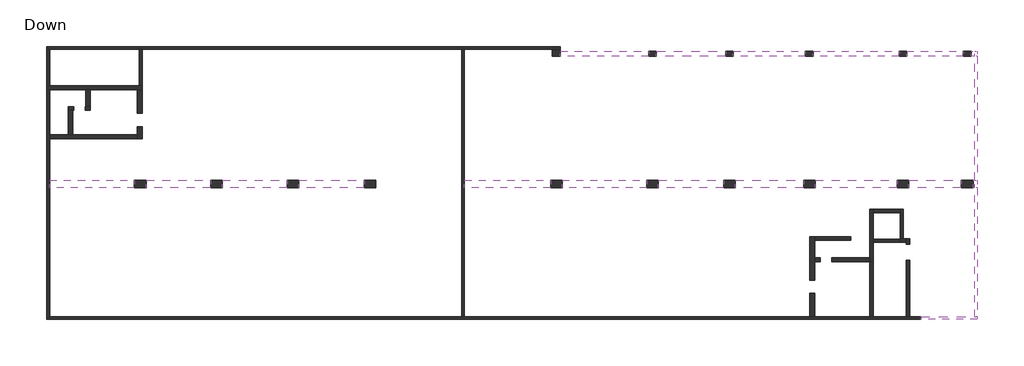
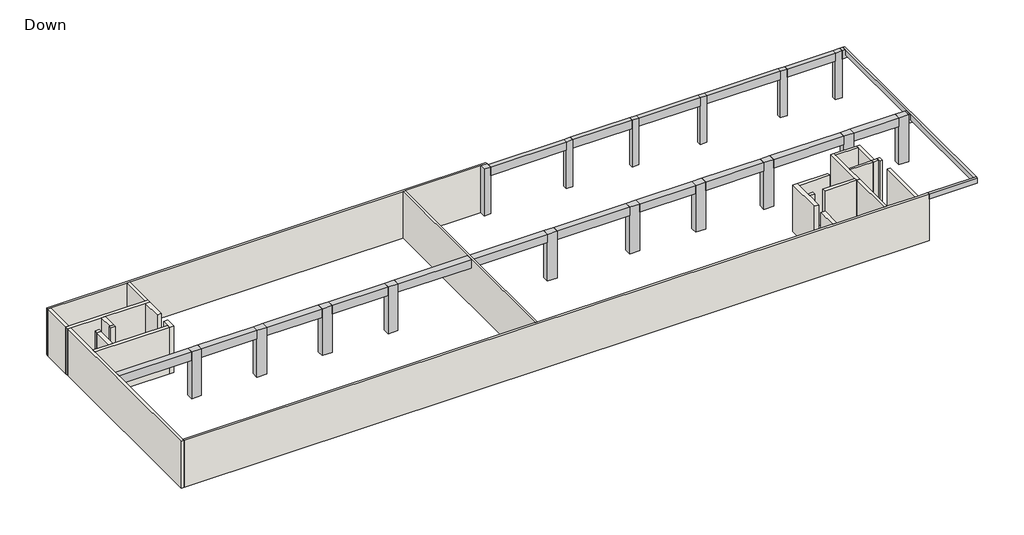
# One storey: 27 walls, 19 beams, 16 columns.
"""IFC4 building model written with IfcOpenShell, lengths in millimetres."""

from ifc_helpers import new_model, si_unit, frame, origin, origin_with_axes, place, context, project, spatial, polyline, outline, extrude, faceted_brep, element, save

model = new_model("IFC4")

# Units and contexts
model_context = context("Model", 3, world=origin())
ifc_project = project(units=[si_unit("LENGTHUNIT", "METRE", prefix="MILLI")], contexts=[model_context])

# Site, building, storey
site = spatial("IfcSite", under=ifc_project)
building = spatial("IfcBuilding", under=site)
storey = spatial("IfcBuildingStorey", under=building, Name="Down", Elevation=0.0)

# Beams
placement = place(None, origin())
element("IfcBeam", 1, ObjectType="Concrete Rectengular Beam : 20/50", at=placement, inside=storey, context=model_context, shape_type="Brep", body=[
    faceted_brep([(30873.6352373, -8183.3289062, 4500.0), (30873.6352373, -8183.3289062, 4000.0), (30873.6352373, -8383.3289062, 4000.0), (30873.6352373, -8383.3289062, 4500.0), (35273.6352373, -8383.3289062, 4500.0), (35273.6352373, -8183.3289062, 4500.0), (35073.6352373, -8183.3289062, 4500.0), (35273.6352373, -8383.3289062, 4000.0), (35073.6352373, -8183.3289062, 4000.0), (35273.6352373, -8183.3289062, 4000.0)], [[[0, 1, 2, 3]], [[0, 3, 4, 5, 6]], [[3, 2, 7, 4]], [[2, 1, 8, 9, 7]], [[1, 0, 6, 5, 9, 8]], [[5, 4, 7, 9]]]),
])
element("IfcBeam", 2, ObjectType="Concrete Rectengular Beam : 20/50", at=placement, inside=storey, context=model_context, shape_type="Brep", body=[
    faceted_brep([(35273.6352373, 12515.9833477, 4500.0), (35073.6352373, 12515.9833477, 4500.0), (35073.6352373, 12115.9833477, 4500.0), (35073.6352373, 2452.6133039, 4500.0), (35073.6352373, 1852.6133039, 4500.0), (35073.6352373, -8183.3289062, 4500.0), (35273.6352373, -8183.3289062, 4500.0), (35273.6352373, 12515.9833477, 4000.0), (35273.6352373, -8183.3289062, 4000.0), (35273.6352373, 1852.6133039, 4000.0), (35273.6352373, 2452.6133039, 4000.0), (35273.6352373, 12115.9833477, 4000.0), (35073.6352373, 12515.9833477, 4000.0), (35073.6352373, -8183.3289062, 4000.0), (35073.6352373, 1852.6133039, 4000.0), (35073.6352373, 2452.6133039, 4000.0), (35073.6352373, 12115.9833477, 4000.0), (35073.6352373, -8183.3289062, 4100.0)], [[[0, 1, 2, 3, 4, 5, 6]], [[7, 0, 6, 8, 9, 10, 11]], [[12, 7, 11, 10, 9, 8, 13, 14, 15, 16]], [[1, 12, 16, 15, 14, 13, 17, 5, 4, 3, 2]], [[1, 0, 7, 12]], [[6, 5, 17, 13, 8]]]),
])
element("IfcBeam", 3, ObjectType="Concrete Rectengular Beam : 40/80", at=placement, inside=storey, context=model_context, shape_type="Brep", body=[
    faceted_brep([(34777.3208435, 12515.9833477, 4500.0), (34777.3208435, 12115.9833477, 4500.0), (35073.6352373, 12115.9833477, 4500.0), (35073.6352373, 12515.9833477, 4500.0), (35273.6352373, 12515.9833477, 3700.0), (34777.3208435, 12515.9833477, 3700.0), (35073.6352373, 12515.9833477, 4000.0), (35273.6352373, 12515.9833477, 4000.0), (35273.6352373, 12115.9833477, 3700.0), (34777.3208435, 12115.9833477, 3700.0), (35273.6352373, 12115.9833477, 4000.0), (35073.6352373, 12115.9833477, 4000.0), (35073.6352373, 12115.9833477, 4100.0), (34777.3208435, 12115.9833477, 4100.0)], [[[0, 1, 2, 3]], [[4, 5, 0, 3, 6, 7]], [[4, 8, 9, 5]], [[9, 8, 10, 11, 12, 2, 1, 13]], [[8, 4, 7, 10]], [[1, 0, 5, 9, 13]], [[6, 11, 10, 7]], [[11, 6, 3, 2, 12]]]),
])
element("IfcBeam", 4, ObjectType="Concrete Rectengular Beam : 40/80", at=placement, inside=storey, context=model_context, shape_type="Brep", body=[
    faceted_brep([(29770.3049975, 12515.9833477, 4500.0), (29770.3049975, 12115.9833477, 4500.0), (34177.3208435, 12115.9833477, 4500.0), (34177.3208435, 12515.9833477, 4500.0), (29770.3049975, 12515.9833477, 3700.0), (34177.3208435, 12515.9833477, 3700.0), (29770.3049975, 12115.9833477, 3700.0), (34177.3208435, 12115.9833477, 3700.0), (29770.3049975, 12115.9833477, 4100.0), (34177.3208435, 12115.9833477, 4100.0)], [[[0, 1, 2, 3]], [[4, 0, 3, 5]], [[6, 4, 5, 7]], [[2, 1, 8, 6, 7, 9]], [[1, 0, 4, 6, 8]], [[3, 2, 9, 7, 5]]]),
])
element("IfcBeam", 5, ObjectType="Concrete Rectengular Beam : 40/80", at=placement, inside=storey, context=model_context, shape_type="Brep", body=[
    faceted_brep([(22477.3114752, 12515.9833477, 4500.0), (22477.3114752, 12115.9833477, 4500.0), (29170.3049975, 12115.9833477, 4500.0), (29170.3049975, 12515.9833477, 4500.0), (22477.3114752, 12515.9833477, 3700.0), (29170.3049975, 12515.9833477, 3700.0), (22477.3114752, 12115.9833477, 3700.0), (29170.3049975, 12115.9833477, 3700.0), (22477.3114752, 12115.9833477, 4100.0), (29170.3049975, 12115.9833477, 4100.0)], [[[0, 1, 2, 3]], [[4, 0, 3, 5]], [[6, 4, 5, 7]], [[2, 1, 8, 6, 7, 9]], [[1, 0, 4, 6, 8]], [[3, 2, 9, 7, 5]]]),
])
element("IfcBeam", 6, ObjectType="Concrete Rectengular Beam : 40/80", at=placement, inside=storey, context=model_context, shape_type="Brep", body=[
    faceted_brep([(21877.3114752, 12115.9833477, 4500.0), (21877.3114752, 12515.9833477, 4500.0), (16270.7293524, 12515.9833477, 4500.0), (16270.7293524, 12115.9833477, 4500.0), (21877.3114752, 12515.9833477, 3700.0), (16270.7293524, 12515.9833477, 3700.0), (21877.3114752, 12115.9833477, 3700.0), (16270.7293524, 12115.9833477, 3700.0), (16270.7293524, 12115.9833477, 4100.0), (21877.3114752, 12115.9833477, 4100.0)], [[[0, 1, 2, 3]], [[1, 4, 5, 2]], [[4, 6, 7, 5]], [[0, 3, 8, 7, 6, 9]], [[1, 0, 9, 6, 4]], [[3, 2, 5, 7, 8]]]),
])
element("IfcBeam", 7, ObjectType="Concrete Rectengular Beam : 40/80", at=placement, inside=storey, context=model_context, shape_type="Brep", body=[
    faceted_brep([(15670.7293524, 12115.9833477, 4500.0), (15670.7293524, 12515.9833477, 4500.0), (10272.0355776, 12515.9833477, 4500.0), (10272.0355776, 12115.9833477, 4500.0), (15670.7293524, 12515.9833477, 3700.0), (10272.0355776, 12515.9833477, 3700.0), (15670.7293524, 12115.9833477, 3700.0), (10272.0355776, 12115.9833477, 3700.0), (10272.0355776, 12115.9833477, 4100.0), (15670.7293524, 12115.9833477, 4100.0)], [[[0, 1, 2, 3]], [[1, 4, 5, 2]], [[4, 6, 7, 5]], [[0, 3, 8, 7, 6, 9]], [[1, 0, 9, 6, 4]], [[3, 2, 5, 7, 8]]]),
])
element("IfcBeam", 8, ObjectType="Concrete Rectengular Beam : 40/80", at=placement, inside=storey, context=model_context, shape_type="Brep", body=[
    faceted_brep([(9672.0355776, 12115.9833477, 4500.0), (9672.0355776, 12515.9833477, 4500.0), (2774.3455353, 12515.9833477, 4500.0), (2774.3455353, 12115.9833477, 4500.0), (9672.0355776, 12515.9833477, 3700.0), (2774.3455353, 12515.9833477, 3700.0), (9672.0355776, 12115.9833477, 3700.0), (2774.3455353, 12115.9833477, 3700.0), (2774.3455353, 12115.9833477, 4100.0), (9672.0355776, 12115.9833477, 4100.0)], [[[0, 1, 2, 3]], [[1, 4, 5, 2]], [[4, 6, 7, 5]], [[0, 3, 8, 7, 6, 9]], [[1, 0, 9, 6, 4]], [[3, 2, 5, 7, 8]]]),
])
element("IfcBeam", 9, ObjectType="Concrete Rectengular Beam : 60/80", at=placement, inside=storey, context=model_context, shape_type="Brep", body=[
    faceted_brep([(34927.3208435, 2452.6133039, 4500.0), (34927.3208435, 1852.6133039, 4500.0), (35073.6352373, 1852.6133039, 4500.0), (35073.6352373, 2452.6133039, 4500.0), (34927.3208435, 1852.6133039, 3700.0), (35273.6352373, 1852.6133039, 3700.0), (35273.6352373, 1852.6133039, 4000.0), (35073.6352373, 1852.6133039, 4000.0), (35073.6352373, 1852.6133039, 4100.0), (35273.6352373, 2452.6133039, 3700.0), (34927.3208435, 2452.6133039, 3700.0), (35073.6352373, 2452.6133039, 4100.0), (35073.6352373, 2452.6133039, 4000.0), (35273.6352373, 2452.6133039, 4000.0)], [[[0, 1, 2, 3]], [[4, 5, 6, 7, 8, 2, 1]], [[9, 5, 4, 10]], [[9, 10, 0, 3, 11, 12, 13]], [[5, 9, 13, 6]], [[1, 0, 10, 4]], [[12, 7, 6, 13]], [[7, 12, 11, 3, 2, 8]]]),
])
element("IfcBeam", 10, ObjectType="Concrete Rectengular Beam : 60/80", at=placement, inside=storey, context=model_context, shape_type="SweptSolid", body=[
    extrude(outline(polyline([(29920.3049975, 1852.6133039), (29920.3049975, 2452.6133039), (34027.3208435, 2452.6133039), (34027.3208435, 1852.6133039), (29920.3049975, 1852.6133039)])), frame((0.0, 0.0, 3700.0), z_axis=(0.0, 0.0, 1.0), x_axis=(1.0, 0.0, 0.0)), (0.0, 0.0, 1.0), 800.0),
])
element("IfcBeam", 11, ObjectType="Concrete Rectengular Beam : 60/80", at=placement, inside=storey, context=model_context, shape_type="SweptSolid", body=[
    extrude(outline(polyline([(29020.3049975, 2452.6133039), (29020.3049975, 1852.6133039), (22627.3114752, 1852.6133039), (22627.3114752, 2452.6133039), (29020.3049975, 2452.6133039)])), frame((0.0, 0.0, 3700.0), z_axis=(0.0, 0.0, 1.0), x_axis=(1.0, 0.0, 0.0)), (0.0, 0.0, 1.0), 800.0),
])
element("IfcBeam", 12, ObjectType="Concrete Rectengular Beam : 60/80", at=placement, inside=storey, context=model_context, shape_type="SweptSolid", body=[
    extrude(outline(polyline([(21727.3114752, 2452.6133039), (21727.3114752, 1852.6133039), (16420.7293524, 1852.6133039), (16420.7293524, 2452.6133039), (21727.3114752, 2452.6133039)])), frame((0.0, 0.0, 3700.0), z_axis=(0.0, 0.0, 1.0), x_axis=(1.0, 0.0, 0.0)), (0.0, 0.0, 1.0), 800.0),
])
element("IfcBeam", 13, ObjectType="Concrete Rectengular Beam : 60/80", at=placement, inside=storey, context=model_context, shape_type="SweptSolid", body=[
    extrude(outline(polyline([(15520.7293524, 2452.6133039), (15520.7293524, 1852.6133039), (10422.0355776, 1852.6133039), (10422.0355776, 2452.6133039), (15520.7293524, 2452.6133039)])), frame((0.0, 0.0, 3700.0), z_axis=(0.0, 0.0, 1.0), x_axis=(1.0, 0.0, 0.0)), (0.0, 0.0, 1.0), 800.0),
])
element("IfcBeam", 14, ObjectType="Concrete Rectengular Beam : 60/80", at=placement, inside=storey, context=model_context, shape_type="SweptSolid", body=[
    extrude(outline(polyline([(9522.0355776, 2452.6133039), (9522.0355776, 1852.6133039), (2924.3455353, 1852.6133039), (2924.3455353, 2452.6133039), (9522.0355776, 2452.6133039)])), frame((0.0, 0.0, 3700.0), z_axis=(0.0, 0.0, 1.0), x_axis=(1.0, 0.0, 0.0)), (0.0, 0.0, 1.0), 800.0),
])
element("IfcBeam", 15, ObjectType="Concrete Rectengular Beam : 60/80", at=placement, inside=storey, context=model_context, shape_type="Brep", body=[
    faceted_brep([(-11589.7528998, 2452.6133039, 4500.0), (-11589.7528998, 1852.6133039, 4500.0), (-4886.1401685, 1852.6133039, 4500.0), (-4886.1401685, 2452.6133039, 4500.0), (-11589.7528998, 2452.6133039, 3700.0), (-4886.1401685, 2452.6133039, 4100.0), (-4886.1401685, 2452.6133039, 3700.0), (-11589.7528998, 1852.6133039, 3700.0), (-4886.1401685, 1852.6133039, 3700.0), (-4886.1401685, 1852.6133039, 4100.0)], [[[0, 1, 2, 3]], [[4, 0, 3, 5, 6]], [[7, 4, 6, 8]], [[1, 7, 8, 9, 2]], [[1, 0, 4, 7]], [[3, 2, 9, 8, 6, 5]]]),
    faceted_brep([(2024.3455353, 2452.6133039, 4500.0), (2024.3455353, 1852.6133039, 4500.0), (2024.3455353, 1852.6133039, 3700.0), (2024.3455353, 2452.6133039, 3700.0), (-4686.1401685, 1852.6133039, 4500.0), (-4686.1401685, 2452.6133039, 4500.0), (-4686.1401685, 2452.6133039, 4100.0), (-4686.1401685, 2452.6133039, 3700.0), (-4686.1401685, 1852.6133039, 3700.0), (-4686.1401685, 1852.6133039, 4100.0)], [[[0, 1, 2, 3]], [[4, 5, 6, 7, 8, 9]], [[1, 0, 5, 4]], [[0, 3, 7, 6, 5]], [[3, 2, 8, 7]], [[2, 1, 4, 9, 8]]]),
])
element("IfcBeam", 16, ObjectType="Concrete Rectengular Beam : 60/80", at=placement, inside=storey, context=model_context, shape_type="SweptSolid", body=[
    extrude(outline(polyline([(-12489.7528998, 2452.6133039), (-12489.7528998, 1852.6133039), (-17591.3777818, 1852.6133039), (-17591.3777818, 2452.6133039), (-12489.7528998, 2452.6133039)])), frame((0.0, 0.0, 3700.0), z_axis=(0.0, 0.0, 1.0), x_axis=(1.0, 0.0, 0.0)), (0.0, 0.0, 1.0), 800.0),
])
element("IfcBeam", 17, ObjectType="Concrete Rectengular Beam : 60/80", at=placement, inside=storey, context=model_context, shape_type="SweptSolid", body=[
    extrude(outline(polyline([(-18491.3777818, 2452.6133039), (-18491.3777818, 1852.6133039), (-23534.5891488, 1852.6133039), (-23534.5891488, 2452.6133039), (-18491.3777818, 2452.6133039)])), frame((0.0, 0.0, 3700.0), z_axis=(0.0, 0.0, 1.0), x_axis=(1.0, 0.0, 0.0)), (0.0, 0.0, 1.0), 800.0),
])
element("IfcBeam", 18, ObjectType="Concrete Rectengular Beam : 60/80", at=placement, inside=storey, context=model_context, shape_type="SweptSolid", body=[
    extrude(outline(polyline([(-24434.5891488, 2452.6133039), (-24434.5891488, 1852.6133039), (-29484.6297539, 1852.6133039), (-29484.6297539, 2452.6133039), (-24434.5891488, 2452.6133039)])), frame((0.0, 0.0, 3700.0), z_axis=(0.0, 0.0, 1.0), x_axis=(1.0, 0.0, 0.0)), (0.0, 0.0, 1.0), 800.0),
])
element("IfcBeam", 19, ObjectType="Concrete Rectengular Beam : 60/80", at=placement, inside=storey, context=model_context, shape_type="Brep", body=[
    faceted_brep([(-30384.6297539, 1852.6133039, 4500.0), (-30384.6297539, 2452.6133039, 4500.0), (-36981.5324359, 2452.6133039, 4500.0), (-36981.5324359, 1852.6133039, 4500.0), (-30384.6297539, 2452.6133039, 3700.0), (-36981.5324359, 2452.6133039, 3700.0), (-36981.5324359, 2452.6133039, 4100.0), (-30384.6297539, 1852.6133039, 3700.0), (-36981.5324359, 1852.6133039, 3700.0), (-36981.5324359, 1852.6133039, 4100.0)], [[[0, 1, 2, 3]], [[1, 4, 5, 6, 2]], [[4, 7, 8, 5]], [[7, 0, 3, 9, 8]], [[1, 0, 7, 4]], [[3, 2, 6, 5, 8, 9]]]),
])

# Columns
element("IfcColumn", 20, ObjectType="Concrete Rectengular Column : 40/60", at=placement, inside=storey, context=model_context, shape_type="SweptSolid", body=[
    extrude(outline(polyline([(21877.3114752, 12515.9833477), (22477.3114752, 12515.9833477), (22477.3114752, 12115.9833477), (21877.3114752, 12115.9833477), (21877.3114752, 12515.9833477)])), origin_with_axes(), (0.0, 0.0, 1.0), 4500.0),
])
element("IfcColumn", 21, ObjectType="Concrete Rectengular Column : 40/60", at=placement, inside=storey, context=model_context, shape_type="SweptSolid", body=[
    extrude(outline(polyline([(15670.7293524, 12515.9833477), (16270.7293524, 12515.9833477), (16270.7293524, 12115.9833477), (15670.7293524, 12115.9833477), (15670.7293524, 12515.9833477)])), origin_with_axes(), (0.0, 0.0, 1.0), 4500.0),
])
element("IfcColumn", 22, ObjectType="Concrete Rectengular Column : 40/60", at=placement, inside=storey, context=model_context, shape_type="SweptSolid", body=[
    extrude(outline(polyline([(9672.0355776, 12515.9833477), (10272.0355776, 12515.9833477), (10272.0355776, 12115.9833477), (9672.0355776, 12115.9833477), (9672.0355776, 12515.9833477)])), origin_with_axes(), (0.0, 0.0, 1.0), 4500.0),
])
element("IfcColumn", 23, ObjectType="Concrete Rectengular Column : 40/60", at=placement, inside=storey, context=model_context, shape_type="SweptSolid", body=[
    extrude(outline(polyline([(29770.3049975, 12115.9833477), (29170.3049975, 12115.9833477), (29170.3049975, 12515.9833477), (29770.3049975, 12515.9833477), (29770.3049975, 12115.9833477)])), origin_with_axes(), (0.0, 0.0, 1.0), 4500.0),
])
element("IfcColumn", 24, ObjectType="Concrete Rectengular Column : 40/60", at=placement, inside=storey, context=model_context, shape_type="SweptSolid", body=[
    extrude(outline(polyline([(34777.3208435, 12115.9833477), (34177.3208435, 12115.9833477), (34177.3208435, 12515.9833477), (34777.3208435, 12515.9833477), (34777.3208435, 12115.9833477)])), origin_with_axes(), (0.0, 0.0, 1.0), 4500.0),
])
element("IfcColumn", 25, ObjectType="Concrete Rectengular Column : 55/60", at=placement, inside=storey, context=model_context, shape_type="Brep", body=[
    faceted_brep([(2174.3455353, 12665.9833477, 0.0), (2774.3455353, 12665.9833477, 0.0), (2774.3455353, 12115.9833477, 0.0), (2174.3455353, 12115.9833477, 0.0), (2174.3455353, 12665.9833477, 4500.0), (2774.3455353, 12665.9833477, 4500.0), (2174.3455353, 12665.9833477, 4100.0), (2774.3455353, 12115.9833477, 4500.0), (2174.3455353, 12115.9833477, 4500.0), (2174.3455353, 12115.9833477, 4100.0)], [[[0, 1, 2, 3]], [[4, 5, 1, 0, 6]], [[5, 7, 2, 1]], [[7, 8, 9, 3, 2]], [[8, 4, 6, 0, 3, 9]], [[4, 8, 7, 5]]]),
])
element("IfcColumn", 26, ObjectType="Concrete Rectengular Column : 60/90", at=placement, inside=storey, context=model_context, shape_type="SweptSolid", body=[
    extrude(outline(polyline([(29020.3049975, 2452.6133039), (29920.3049975, 2452.6133039), (29920.3049975, 1852.6133039), (29020.3049975, 1852.6133039), (29020.3049975, 2452.6133039)])), origin_with_axes(), (0.0, 0.0, 1.0), 4500.0),
])
element("IfcColumn", 27, ObjectType="Concrete Rectengular Column : 60/90", at=placement, inside=storey, context=model_context, shape_type="SweptSolid", body=[
    extrude(outline(polyline([(34027.3208435, 2452.6133039), (34927.3208435, 2452.6133039), (34927.3208435, 1852.6133039), (34027.3208435, 1852.6133039), (34027.3208435, 2452.6133039)])), origin_with_axes(), (0.0, 0.0, 1.0), 4500.0),
])
element("IfcColumn", 28, ObjectType="Concrete Rectengular Column : 60/90", at=placement, inside=storey, context=model_context, shape_type="SweptSolid", body=[
    extrude(outline(polyline([(21727.3114752, 2452.6133039), (22627.3114752, 2452.6133039), (22627.3114752, 1852.6133039), (21727.3114752, 1852.6133039), (21727.3114752, 2452.6133039)])), origin_with_axes(), (0.0, 0.0, 1.0), 4500.0),
])
element("IfcColumn", 29, ObjectType="Concrete Rectengular Column : 60/90", at=placement, inside=storey, context=model_context, shape_type="SweptSolid", body=[
    extrude(outline(polyline([(15520.7293524, 2452.6133039), (16420.7293524, 2452.6133039), (16420.7293524, 1852.6133039), (15520.7293524, 1852.6133039), (15520.7293524, 2452.6133039)])), origin_with_axes(), (0.0, 0.0, 1.0), 4500.0),
])
element("IfcColumn", 30, ObjectType="Concrete Rectengular Column : 60/90", at=placement, inside=storey, context=model_context, shape_type="SweptSolid", body=[
    extrude(outline(polyline([(9522.0355776, 2452.6133039), (10422.0355776, 2452.6133039), (10422.0355776, 1852.6133039), (9522.0355776, 1852.6133039), (9522.0355776, 2452.6133039)])), origin_with_axes(), (0.0, 0.0, 1.0), 4500.0),
])
element("IfcColumn", 31, ObjectType="Concrete Rectengular Column : 60/90", at=placement, inside=storey, context=model_context, shape_type="SweptSolid", body=[
    extrude(outline(polyline([(2024.3455353, 2452.6133039), (2924.3455353, 2452.6133039), (2924.3455353, 1852.6133039), (2024.3455353, 1852.6133039), (2024.3455353, 2452.6133039)])), origin_with_axes(), (0.0, 0.0, 1.0), 4500.0),
])
element("IfcColumn", 32, ObjectType="Concrete Rectengular Column : 60/90", at=placement, inside=storey, context=model_context, shape_type="SweptSolid", body=[
    extrude(outline(polyline([(-12489.7528998, 2452.6133039), (-11589.7528998, 2452.6133039), (-11589.7528998, 1852.6133039), (-12489.7528998, 1852.6133039), (-12489.7528998, 2452.6133039)])), origin_with_axes(), (0.0, 0.0, 1.0), 4500.0),
])
element("IfcColumn", 33, ObjectType="Concrete Rectengular Column : 60/90", at=placement, inside=storey, context=model_context, shape_type="SweptSolid", body=[
    extrude(outline(polyline([(-18491.3777818, 2452.6133039), (-17591.3777818, 2452.6133039), (-17591.3777818, 1852.6133039), (-18491.3777818, 1852.6133039), (-18491.3777818, 2452.6133039)])), origin_with_axes(), (0.0, 0.0, 1.0), 4500.0),
])
element("IfcColumn", 34, ObjectType="Concrete Rectengular Column : 60/90", at=placement, inside=storey, context=model_context, shape_type="SweptSolid", body=[
    extrude(outline(polyline([(-24434.5891488, 2452.6133039), (-23534.5891488, 2452.6133039), (-23534.5891488, 1852.6133039), (-24434.5891488, 1852.6133039), (-24434.5891488, 2452.6133039)])), origin_with_axes(), (0.0, 0.0, 1.0), 4500.0),
])
element("IfcColumn", 35, ObjectType="Concrete Rectengular Column : 60/90", at=placement, inside=storey, context=model_context, shape_type="SweptSolid", body=[
    extrude(outline(polyline([(-30384.6297539, 2452.6133039), (-29484.6297539, 2452.6133039), (-29484.6297539, 1852.6133039), (-30384.6297539, 1852.6133039), (-30384.6297539, 2452.6133039)])), origin_with_axes(), (0.0, 0.0, 1.0), 4500.0),
])

# Walls
element("IfcWall", 36, ObjectType="20", at=placement, inside=storey, context=model_context, shape_type="Brep", body=[
    faceted_brep([(2774.3455353, 12865.9833477, 0.0), (-37231.5324359, 12865.9833477, 0.0), (-37231.5324359, 12865.9833477, 4500.0), (2774.3455353, 12865.9833477, 4500.0), (2774.3455353, 12665.9833477, 0.0), (2774.3455353, 12665.9833477, 4500.0), (2174.3455353, 12665.9833477, 4500.0), (-4686.1401685, 12665.9833477, 4500.0), (-4886.1401685, 12665.9833477, 4500.0), (-29780.4573498, 12665.9833477, 4500.0), (-30010.4573498, 12665.9833477, 4500.0), (-36981.5324359, 12665.9833477, 4500.0), (-37231.5324359, 12665.9833477, 4500.0), (-37231.5324359, 12665.9833477, 0.0), (-36981.5324359, 12665.9833477, 0.0), (-30010.4573498, 12665.9833477, 0.0), (-29780.4573498, 12665.9833477, 0.0), (-4886.1401685, 12665.9833477, 0.0), (-4686.1401685, 12665.9833477, 0.0), (2174.3455353, 12665.9833477, 0.0)], [[[0, 1, 2, 3]], [[4, 5, 6, 7, 8, 9, 10, 11, 12, 13, 14, 15, 16, 17, 18, 19]], [[1, 0, 4, 19, 18, 17, 16, 15, 14, 13]], [[3, 2, 12, 11, 10, 9, 8, 7, 6, 5]], [[0, 3, 5, 4]], [[2, 1, 13, 12]]]),
])
element("IfcWall", 37, ObjectType="20", at=placement, inside=storey, context=model_context, shape_type="Brep", body=[
    faceted_brep([(-36981.5324359, -8383.3289062, 0.0), (30873.6352373, -8383.3289062, 0.0), (30873.6352373, -8383.3289062, 4000.0), (30873.6352373, -8383.3289062, 4500.0), (-36981.5324359, -8383.3289062, 4500.0), (-36981.5324359, -8183.3289062, 0.0), (-36981.5324359, -8183.3289062, 4100.0), (-36981.5324359, -8183.3289062, 4500.0), (-4886.1401685, -8183.3289062, 4500.0), (-4686.1401685, -8183.3289062, 4500.0), (22192.8106957, -8183.3289062, 4500.0), (22592.8106957, -8183.3289062, 4500.0), (26893.3884, -8183.3289062, 4500.0), (27143.3884, -8183.3289062, 4500.0), (29744.7199004, -8183.3289062, 4500.0), (29994.7199004, -8183.3289062, 4500.0), (30873.6352373, -8183.3289062, 4500.0), (30873.6352373, -8183.3289062, 4000.0), (30873.6352373, -8183.3289062, 0.0), (29994.7199004, -8183.3289062, 0.0), (29744.7199004, -8183.3289062, 0.0), (27143.3884, -8183.3289062, 0.0), (26893.3884, -8183.3289062, 0.0), (22592.8106957, -8183.3289062, 0.0), (22192.8106957, -8183.3289062, 0.0), (-4686.1401685, -8183.3289062, 0.0), (-4886.1401685, -8183.3289062, 0.0)], [[[0, 1, 2, 3, 4]], [[5, 6, 7, 8, 9, 10, 11, 12, 13, 14, 15, 16, 17, 18, 19, 20, 21, 22, 23, 24, 25, 26]], [[1, 0, 5, 26, 25, 24, 23, 22, 21, 20, 19, 18]], [[3, 2, 1, 18, 17, 16]], [[4, 3, 16, 15, 14, 13, 12, 11, 10, 9, 8, 7]], [[0, 4, 7, 6, 5]]]),
])
element("IfcWall", 38, ObjectType="20", at=placement, inside=storey, context=model_context, shape_type="SweptSolid", body=[
    extrude(outline(polyline([(27139.9357672, -2160.3079756), (29245.3524403, -2160.3079756), (29245.3524403, -2360.3079756), (27139.9357672, -2360.3079756), (27139.9357672, -2160.3079756)])), origin_with_axes(), (0.0, 0.0, 1.0), 4500.0),
])
element("IfcWall", 39, ObjectType="20", at=placement, inside=storey, context=model_context, shape_type="Brep", body=[
    faceted_brep([(-4886.1401685, 12665.9833477, 0.0), (-4886.1401685, -8183.3289062, 0.0), (-4886.1401685, -8183.3289062, 4100.0), (-4886.1401685, -8183.3289062, 4500.0), (-4886.1401685, 1852.6133039, 4500.0), (-4886.1401685, 2452.6133039, 4500.0), (-4886.1401685, 12665.9833477, 4500.0), (-4886.1401685, 12665.9833477, 4100.0), (-4686.1401685, 12665.9833477, 0.0), (-4686.1401685, 12665.9833477, 4100.0), (-4686.1401685, 12665.9833477, 4500.0), (-4686.1401685, 2452.6133039, 4500.0), (-4686.1401685, 1852.6133039, 4500.0), (-4686.1401685, -8183.3289062, 4500.0), (-4686.1401685, -8183.3289062, 4100.0), (-4686.1401685, -8183.3289062, 0.0)], [[[0, 1, 2, 3, 4, 5, 6, 7]], [[8, 9, 10, 11, 12, 13, 14, 15]], [[1, 0, 8, 15]], [[6, 5, 4, 3, 13, 12, 11, 10]], [[0, 7, 6, 10, 9, 8]], [[3, 2, 1, 15, 14, 13]]]),
])
element("IfcWall", 40, ObjectType="23", at=placement, inside=storey, context=model_context, shape_type="Brep", body=[
    faceted_brep([(-30010.4573498, 12665.9833477, 0.0), (-30010.4573498, 9800.978884, 0.0), (-30010.4573498, 9800.978884, 4500.0), (-30010.4573498, 12665.9833477, 4500.0), (-29780.4573498, 12665.9833477, 0.0), (-29780.4573498, 12665.9833477, 4100.0), (-29780.4573498, 12665.9833477, 4500.0), (-29780.4573498, 9800.978884, 4500.0), (-29780.4573498, 9800.978884, 0.0)], [[[0, 1, 2, 3]], [[4, 5, 6, 7, 8]], [[1, 0, 4, 8]], [[3, 2, 7, 6]], [[0, 3, 6, 5, 4]], [[2, 1, 8, 7]]]),
])
element("IfcWall", 41, ObjectType="25", at=placement, inside=storey, context=model_context, shape_type="SweptSolid", body=[
    extrude(outline(polyline([(-36981.5324359, 12665.9833477), (-36981.5324359, 9800.978884), (-37231.5324359, 9800.978884), (-37231.5324359, 12665.9833477), (-36981.5324359, 12665.9833477)])), origin_with_axes(), (0.0, 0.0, 1.0), 4500.0),
])
element("IfcWall", 42, ObjectType="25", at=placement, inside=storey, context=model_context, shape_type="Brep", body=[
    faceted_brep([(-37231.5324359, 9500.978884, 0.0), (-37231.5324359, -8383.3289062, 0.0), (-37231.5324359, -8383.3289062, 4500.0), (-37231.5324359, 9500.978884, 4500.0), (-36981.5324359, 9500.978884, 0.0), (-36981.5324359, 9500.978884, 4250.0), (-36981.5324359, 9500.978884, 4500.0), (-36981.5324359, 5997.6022486, 4500.0), (-36981.5324359, 5697.6022486, 4500.0), (-36981.5324359, 2452.6133039, 4500.0), (-36981.5324359, 1852.6133039, 4500.0), (-36981.5324359, -8183.3289062, 4500.0), (-36981.5324359, -8383.3289062, 4500.0), (-36981.5324359, -8383.3289062, 0.0), (-36981.5324359, -8183.3289062, 0.0), (-36981.5324359, 5697.6022486, 0.0), (-36981.5324359, 5997.6022486, 0.0)], [[[0, 1, 2, 3]], [[4, 5, 6, 7, 8, 9, 10, 11, 12, 13, 14, 15, 16]], [[1, 0, 4, 16, 15, 14, 13]], [[3, 2, 12, 11, 10, 9, 8, 7, 6]], [[0, 3, 6, 5, 4]], [[2, 1, 13, 12]]]),
])
element("IfcWall", 43, ObjectType="25", at=placement, inside=storey, context=model_context, shape_type="Brep", body=[
    faceted_brep([(29994.7199004, -8183.3289062, 0.0), (29994.7199004, -3766.5105737, 0.0), (29994.7199004, -3766.5105737, 4100.0), (29994.7199004, -3766.5105737, 4500.0), (29994.7199004, -8183.3289062, 4500.0), (29994.7199004, -8183.3289062, 4100.0), (29744.7199004, -8183.3289062, 0.0), (29744.7199004, -8183.3289062, 4500.0), (29744.7199004, -3766.5105737, 4500.0), (29744.7199004, -3766.5105737, 4100.0), (29744.7199004, -3766.5105737, 0.0)], [[[0, 1, 2, 3, 4, 5]], [[6, 7, 8, 9, 10]], [[1, 0, 6, 10]], [[3, 2, 1, 10, 9, 8]], [[4, 3, 8, 7]], [[0, 5, 4, 7, 6]]]),
])
element("IfcWall", 44, ObjectType="25", at=placement, inside=storey, context=model_context, shape_type="Brep", body=[
    faceted_brep([(29994.7199004, -2514.5866947, 0.0), (29994.7199004, -2110.3079756, 0.0), (29994.7199004, -2110.3079756, 4100.0), (29994.7199004, -2110.3079756, 4500.0), (29994.7199004, -2514.5866947, 4500.0), (29994.7199004, -2514.5866947, 4100.0), (29744.7199004, -2514.5866947, 0.0), (29744.7199004, -2514.5866947, 4100.0), (29744.7199004, -2514.5866947, 4500.0), (29744.7199004, -2360.3079756, 4500.0), (29744.7199004, -2110.3079756, 4500.0), (29744.7199004, -2110.3079756, 0.0), (29744.7199004, -2360.3079756, 0.0)], [[[0, 1, 2, 3, 4, 5]], [[6, 7, 8, 9, 10, 11, 12]], [[1, 0, 6, 12, 11]], [[4, 3, 10, 9, 8]], [[0, 5, 4, 8, 7, 6]], [[3, 2, 1, 11, 10]]]),
])
element("IfcWall", 45, ObjectType="25", at=placement, inside=storey, context=model_context, shape_type="Brep", body=[
    faceted_brep([(29744.7199004, -2110.3079756, 0.0), (29495.5138576, -2110.3079756, 0.0), (29245.5138576, -2110.3079756, 0.0), (29245.3524403, -2110.3079756, 0.0), (29245.3524403, -2110.3079756, 4500.0), (29245.5138576, -2110.3079756, 4500.0), (29495.5138576, -2110.3079756, 4500.0), (29744.7199004, -2110.3079756, 4500.0), (29744.7199004, -2360.3079756, 0.0), (29744.7199004, -2360.3079756, 4500.0), (29245.3524403, -2360.3079756, 4500.0), (29245.3524403, -2360.3079756, 0.0), (29245.3524403, -2160.3079756, 0.0), (29245.3524403, -2160.3079756, 4500.0)], [[[0, 1, 2, 3, 4, 5, 6, 7]], [[8, 9, 10, 11]], [[3, 2, 1, 0, 8, 11, 12]], [[4, 3, 12, 11, 10, 13]], [[7, 6, 5, 4, 13, 10, 9]], [[0, 7, 9, 8]]]),
])
element("IfcWall", 46, ObjectType="25", at=placement, inside=storey, context=model_context, shape_type="Brep", body=[
    faceted_brep([(29495.5138576, -2110.3079756, 0.0), (29495.5138576, 189.1668387, 0.0), (29495.5138576, 189.1668387, 4100.0), (29495.5138576, 189.1668387, 4500.0), (29495.5138576, -2110.3079756, 4500.0), (29495.5138576, -2110.3079756, 4100.0), (29245.5138576, -2110.3079756, 0.0), (29245.5138576, -2110.3079756, 4500.0), (29245.5138576, -60.8331613, 4500.0), (29245.5138576, 189.1668387, 4500.0), (29245.5138576, 189.1668387, 0.0), (29245.5138576, -60.8331613, 0.0)], [[[0, 1, 2, 3, 4, 5]], [[6, 7, 8, 9, 10, 11]], [[1, 0, 6, 11, 10]], [[4, 3, 9, 8, 7]], [[0, 5, 4, 7, 6]], [[3, 2, 1, 10, 9]]]),
])
element("IfcWall", 47, ObjectType="25", at=placement, inside=storey, context=model_context, shape_type="SweptSolid", body=[
    extrude(outline(polyline([(27139.9357672, 189.1668387), (29245.5138576, 189.1668387), (29245.5138576, -60.8331613), (27139.9357672, -60.8331613), (27139.9357672, 189.1668387)])), origin_with_axes(), (0.0, 0.0, 1.0), 4500.0),
])
element("IfcWall", 48, ObjectType="25", at=placement, inside=storey, context=model_context, shape_type="Brep", body=[
    faceted_brep([(26893.3884, -3883.3566788, 0.0), (26893.3884, -8183.3289062, 0.0), (26893.3884, -8183.3289062, 4250.0), (26893.3884, -8183.3289062, 4500.0), (26893.3884, -3883.3566788, 4500.0), (26893.3884, -3883.3566788, 4250.0), (27143.3884, -3883.3566788, 0.0), (27143.3884, -3883.3566788, 4500.0), (27143.3884, -8183.3289062, 4500.0), (27143.3884, -8183.3289062, 0.0), (27139.9357672, -3883.3566788, 0.0), (27139.9357672, -3883.3566788, 4500.0)], [[[0, 1, 2, 3, 4, 5]], [[6, 7, 8, 9]], [[1, 0, 10, 6, 9]], [[4, 3, 8, 7, 11]], [[0, 5, 4, 11, 7, 6, 10]], [[3, 2, 1, 9, 8]]]),
])
element("IfcWall", 49, ObjectType="27", at=placement, inside=storey, context=model_context, shape_type="Brep", body=[
    faceted_brep([(26869.9357672, 189.1668387, 0.0), (26869.9357672, -3583.3566788, 0.0), (26869.9357672, -3883.3566788, 0.0), (26869.9357672, -3883.3566788, 4500.0), (26869.9357672, -3583.3566788, 4500.0), (26869.9357672, -1932.7380409, 4500.0), (26869.9357672, 189.1668387, 4500.0), (26869.9357672, 189.1668387, 4100.0), (27139.9357672, 189.1668387, 0.0), (27139.9357672, 189.1668387, 4500.0), (27139.9357672, -60.8331613, 4500.0), (27139.9357672, -2160.3079756, 4500.0), (27139.9357672, -2360.3079756, 4500.0), (27139.9357672, -3883.3566788, 4500.0), (27139.9357672, -3883.3566788, 0.0), (27139.9357672, -2360.3079756, 0.0), (27139.9357672, -2160.3079756, 0.0), (27139.9357672, -60.8331613, 0.0), (26893.3884, -3883.3566788, 0.0), (26893.3884, -3883.3566788, 4500.0)], [[[0, 1, 2, 3, 4, 5, 6, 7]], [[8, 9, 10, 11, 12, 13, 14, 15, 16, 17]], [[2, 1, 0, 8, 17, 16, 15, 14, 18]], [[6, 5, 4, 3, 19, 13, 12, 11, 10, 9]], [[0, 7, 6, 9, 8]], [[3, 2, 18, 14, 13, 19]]]),
])
element("IfcWall", 50, ObjectType="27", at=placement, inside=storey, context=model_context, shape_type="Brep", body=[
    faceted_brep([(-35525.2356133, 7897.529186, 0.0), (-35175.2356133, 7897.529186, 0.0), (-35131.0080225, 7897.529186, 0.0), (-35131.0080225, 7897.529186, 4250.0), (-35131.0080225, 7897.529186, 4500.0), (-35175.2356133, 7897.529186, 4500.0), (-35525.2356133, 7897.529186, 4500.0), (-35525.2356133, 8167.529186, 0.0), (-35525.2356133, 8167.529186, 4250.0), (-35525.2356133, 8167.529186, 4500.0), (-35131.0080225, 8167.529186, 4500.0), (-35131.0080225, 8167.529186, 4250.0), (-35131.0080225, 8167.529186, 0.0)], [[[0, 1, 2, 3, 4, 5, 6]], [[7, 8, 9, 10, 11, 12]], [[2, 1, 0, 7, 12]], [[4, 3, 2, 12, 11, 10]], [[6, 5, 4, 10, 9]], [[0, 6, 9, 8, 7]]]),
])
element("IfcWall", 51, ObjectType="27", at=placement, inside=storey, context=model_context, shape_type="Brep", body=[
    faceted_brep([(-34230.8736368, 7897.529186, 0.0), (-33829.9452937, 7897.529186, 0.0), (-33829.9452937, 7897.529186, 4250.0), (-33829.9452937, 7897.529186, 4500.0), (-34230.8736368, 7897.529186, 4500.0), (-34230.8736368, 7897.529186, 4250.0), (-34230.8736368, 8167.529186, 0.0), (-34230.8736368, 8167.529186, 4250.0), (-34230.8736368, 8167.529186, 4500.0), (-34179.9452937, 8167.529186, 4500.0), (-33829.9452937, 8167.529186, 4500.0), (-33829.9452937, 8167.529186, 0.0), (-34179.9452937, 8167.529186, 0.0)], [[[0, 1, 2, 3, 4, 5]], [[6, 7, 8, 9, 10, 11, 12]], [[1, 0, 6, 12, 11]], [[4, 3, 10, 9, 8]], [[0, 5, 4, 8, 7, 6]], [[3, 2, 1, 11, 10]]]),
])
element("IfcWall", 52, ObjectType="30", at=placement, inside=storey, context=model_context, shape_type="Brep", body=[
    faceted_brep([(-29780.4573498, 9800.978884, 0.0), (-30010.4573498, 9800.978884, 0.0), (-36981.5324359, 9800.978884, 0.0), (-37231.5324359, 9800.978884, 0.0), (-37231.5324359, 9800.978884, 4500.0), (-36981.5324359, 9800.978884, 4500.0), (-30010.4573498, 9800.978884, 4500.0), (-29780.4573498, 9800.978884, 4500.0), (-29780.4573498, 9500.978884, 0.0), (-29780.4573498, 9500.978884, 4500.0), (-30180.4573498, 9500.978884, 4500.0), (-33829.9452937, 9500.978884, 4500.0), (-34179.9452937, 9500.978884, 4500.0), (-36981.5324359, 9500.978884, 4500.0), (-37231.5324359, 9500.978884, 4500.0), (-37231.5324359, 9500.978884, 0.0), (-36981.5324359, 9500.978884, 0.0), (-34179.9452937, 9500.978884, 0.0), (-33829.9452937, 9500.978884, 0.0), (-30180.4573498, 9500.978884, 0.0)], [[[0, 1, 2, 3, 4, 5, 6, 7]], [[8, 9, 10, 11, 12, 13, 14, 15, 16, 17, 18, 19]], [[3, 2, 1, 0, 8, 19, 18, 17, 16, 15]], [[7, 6, 5, 4, 14, 13, 12, 11, 10, 9]], [[4, 3, 15, 14]], [[0, 7, 9, 8]]]),
])
element("IfcWall", 53, ObjectType="30", at=placement, inside=storey, context=model_context, shape_type="Brep", body=[
    faceted_brep([(25386.8359355, -1932.7380409, 0.0), (22592.8106957, -1932.7380409, 0.0), (22592.8106957, -1932.7380409, 4500.0), (25386.8359355, -1932.7380409, 4500.0), (25386.8359355, -1932.7380409, 4250.0), (25386.8359355, -2232.7380409, 0.0), (25386.8359355, -2232.7380409, 4250.0), (25386.8359355, -2232.7380409, 4500.0), (22592.8106957, -2232.7380409, 4500.0), (22592.8106957, -2232.7380409, 4250.0), (22592.8106957, -2232.7380409, 0.0)], [[[0, 1, 2, 3, 4]], [[5, 6, 7, 8, 9, 10]], [[1, 0, 5, 10]], [[3, 2, 8, 7]], [[0, 4, 3, 7, 6, 5]], [[2, 1, 10, 9, 8]]]),
])
element("IfcWall", 54, ObjectType="30", at=placement, inside=storey, context=model_context, shape_type="Brep", body=[
    faceted_brep([(22592.8106957, -3883.3566788, 0.0), (23037.1054794, -3883.3566788, 0.0), (23037.1054794, -3883.3566788, 4250.0), (23037.1054794, -3883.3566788, 4500.0), (22592.8106957, -3883.3566788, 4500.0), (22592.8106957, -3883.3566788, 4250.0), (22592.8106957, -3583.3566788, 0.0), (22592.8106957, -3583.3566788, 4250.0), (22592.8106957, -3583.3566788, 4500.0), (23037.1054794, -3583.3566788, 4500.0), (23037.1054794, -3583.3566788, 4250.0), (23037.1054794, -3583.3566788, 0.0), (23037.1054794, -3733.3566788, 4500.0)], [[[0, 1, 2, 3, 4, 5]], [[6, 7, 8, 9, 10, 11]], [[1, 0, 6, 11]], [[3, 2, 1, 11, 10, 9, 12]], [[4, 3, 12, 9, 8]], [[0, 5, 4, 8, 7, 6]]]),
])
element("IfcWall", 55, ObjectType="30", at=placement, inside=storey, context=model_context, shape_type="Brep", body=[
    faceted_brep([(23943.9406174, -3883.3566788, 0.0), (26869.9357672, -3883.3566788, 0.0), (26869.9357672, -3883.3566788, 4500.0), (23943.9406174, -3883.3566788, 4500.0), (23943.9406174, -3883.3566788, 4250.0), (23943.9406174, -3583.3566788, 0.0), (23943.9406174, -3583.3566788, 4250.0), (23943.9406174, -3583.3566788, 4500.0), (26869.9357672, -3583.3566788, 4500.0), (26869.9357672, -3583.3566788, 4250.0), (26869.9357672, -3583.3566788, 0.0), (23943.9406174, -3733.3566788, 4500.0)], [[[0, 1, 2, 3, 4]], [[5, 6, 7, 8, 9, 10]], [[1, 0, 5, 10]], [[3, 2, 8, 7, 11]], [[0, 4, 3, 11, 7, 6, 5]], [[2, 1, 10, 9, 8]]]),
])
element("IfcWall", 56, ObjectType="30", at=placement, inside=storey, context=model_context, shape_type="Brep", body=[
    faceted_brep([(-36981.5324359, 5697.6022486, 0.0), (-30180.4573498, 5697.6022486, 0.0), (-30180.4573498, 5697.6022486, 4500.0), (-36981.5324359, 5697.6022486, 4500.0), (-36981.5324359, 5697.6022486, 4100.0), (-36981.5324359, 5997.6022486, 0.0), (-36981.5324359, 5997.6022486, 4250.0), (-36981.5324359, 5997.6022486, 4500.0), (-35525.2356133, 5997.6022486, 4500.0), (-35175.2356133, 5997.6022486, 4500.0), (-30180.4573498, 5997.6022486, 4500.0), (-30180.4573498, 5997.6022486, 4250.0), (-30180.4573498, 5997.6022486, 0.0), (-35175.2356133, 5997.6022486, 0.0), (-35525.2356133, 5997.6022486, 0.0)], [[[0, 1, 2, 3, 4]], [[5, 6, 7, 8, 9, 10, 11, 12, 13, 14]], [[1, 0, 5, 14, 13, 12]], [[3, 2, 10, 9, 8, 7]], [[0, 4, 3, 7, 6, 5]], [[2, 1, 12, 11, 10]]]),
])
element("IfcWall", 57, ObjectType="35", at=placement, inside=storey, context=model_context, shape_type="Brep", body=[
    faceted_brep([(-35175.2356133, 5997.6022486, 0.0), (-35175.2356133, 7897.529186, 0.0), (-35175.2356133, 7897.529186, 4250.0), (-35175.2356133, 7897.529186, 4500.0), (-35175.2356133, 5997.6022486, 4500.0), (-35175.2356133, 5997.6022486, 4250.0), (-35525.2356133, 5997.6022486, 0.0), (-35525.2356133, 5997.6022486, 4250.0), (-35525.2356133, 5997.6022486, 4500.0), (-35525.2356133, 7897.529186, 4500.0), (-35525.2356133, 7897.529186, 0.0)], [[[0, 1, 2, 3, 4, 5]], [[6, 7, 8, 9, 10]], [[1, 0, 6, 10]], [[4, 3, 9, 8]], [[0, 5, 4, 8, 7, 6]], [[3, 2, 1, 10, 9]]]),
])
element("IfcWall", 58, ObjectType="35", at=placement, inside=storey, context=model_context, shape_type="Brep", body=[
    faceted_brep([(-33829.9452937, 8167.529186, 0.0), (-33829.9452937, 9500.978884, 0.0), (-33829.9452937, 9500.978884, 4250.0), (-33829.9452937, 9500.978884, 4500.0), (-33829.9452937, 8167.529186, 4500.0), (-34179.9452937, 8167.529186, 0.0), (-34179.9452937, 8167.529186, 4250.0), (-34179.9452937, 8167.529186, 4500.0), (-34179.9452937, 9500.978884, 4500.0), (-34179.9452937, 9500.978884, 4250.0), (-34179.9452937, 9500.978884, 0.0)], [[[0, 1, 2, 3, 4]], [[5, 6, 7, 8, 9, 10]], [[1, 0, 5, 10]], [[4, 3, 8, 7]], [[0, 4, 7, 6, 5]], [[3, 2, 1, 10, 9, 8]]]),
])
element("IfcWall", 59, ObjectType="40", at=placement, inside=storey, context=model_context, shape_type="Brep", body=[
    faceted_brep([(22192.8106957, -1932.7380409, 0.0), (22192.8106957, -5323.3186801, 0.0), (22192.8106957, -5323.3186801, 4100.0), (22192.8106957, -5323.3186801, 4500.0), (22192.8106957, -1932.7380409, 4500.0), (22192.8106957, -1932.7380409, 4100.0), (22592.8106957, -1932.7380409, 0.0), (22592.8106957, -1932.7380409, 4500.0), (22592.8106957, -2232.7380409, 4500.0), (22592.8106957, -3583.3566788, 4500.0), (22592.8106957, -3883.3566788, 4500.0), (22592.8106957, -5323.3186801, 4500.0), (22592.8106957, -5323.3186801, 4100.0), (22592.8106957, -5323.3186801, 0.0), (22592.8106957, -3883.3566788, 0.0), (22592.8106957, -3583.3566788, 0.0), (22592.8106957, -2232.7380409, 0.0)], [[[0, 1, 2, 3, 4, 5]], [[6, 7, 8, 9, 10, 11, 12, 13, 14, 15, 16]], [[1, 0, 6, 16, 15, 14, 13]], [[3, 2, 1, 13, 12, 11]], [[4, 3, 11, 10, 9, 8, 7]], [[0, 5, 4, 7, 6]]]),
])
element("IfcWall", 60, ObjectType="40", at=placement, inside=storey, context=model_context, shape_type="Brep", body=[
    faceted_brep([(22192.8106957, -6342.9498143, 0.0), (22192.8106957, -8183.3289062, 0.0), (22192.8106957, -8183.3289062, 4100.0), (22192.8106957, -8183.3289062, 4500.0), (22192.8106957, -6342.9498143, 4500.0), (22192.8106957, -6342.9498143, 4100.0), (22592.8106957, -6342.9498143, 0.0), (22592.8106957, -6342.9498143, 4100.0), (22592.8106957, -6342.9498143, 4500.0), (22592.8106957, -8183.3289062, 4500.0), (22592.8106957, -8183.3289062, 4250.0), (22592.8106957, -8183.3289062, 0.0)], [[[0, 1, 2, 3, 4, 5]], [[6, 7, 8, 9, 10, 11]], [[1, 0, 6, 11]], [[4, 3, 9, 8]], [[0, 5, 4, 8, 7, 6]], [[3, 2, 1, 11, 10, 9]]]),
])
element("IfcWall", 61, ObjectType="40", at=placement, inside=storey, context=model_context, shape_type="Brep", body=[
    faceted_brep([(-29780.4573498, 5697.6022486, 0.0), (-29780.4573498, 6627.4729602, 0.0), (-29780.4573498, 6627.4729602, 4100.0), (-29780.4573498, 6627.4729602, 4500.0), (-29780.4573498, 5697.6022486, 4500.0), (-29780.4573498, 5697.6022486, 4100.0), (-30180.4573498, 5697.6022486, 0.0), (-30180.4573498, 5697.6022486, 4500.0), (-30180.4573498, 5997.6022486, 4500.0), (-30180.4573498, 6627.4729602, 4500.0), (-30180.4573498, 6627.4729602, 4100.0), (-30180.4573498, 6627.4729602, 0.0), (-30180.4573498, 5997.6022486, 0.0)], [[[0, 1, 2, 3, 4, 5]], [[6, 7, 8, 9, 10, 11, 12]], [[1, 0, 6, 12, 11]], [[3, 2, 1, 11, 10, 9]], [[4, 3, 9, 8, 7]], [[0, 5, 4, 7, 6]]]),
])
element("IfcWall", 62, ObjectType="40", at=placement, inside=storey, context=model_context, shape_type="Brep", body=[
    faceted_brep([(-29780.4573498, 7652.6880547, 0.0), (-29780.4573498, 9500.978884, 0.0), (-29780.4573498, 9500.978884, 4500.0), (-29780.4573498, 7652.6880547, 4500.0), (-29780.4573498, 7652.6880547, 4100.0), (-30180.4573498, 7652.6880547, 0.0), (-30180.4573498, 7652.6880547, 4100.0), (-30180.4573498, 7652.6880547, 4500.0), (-30180.4573498, 9500.978884, 4500.0), (-30180.4573498, 9500.978884, 4250.0), (-30180.4573498, 9500.978884, 0.0)], [[[0, 1, 2, 3, 4]], [[5, 6, 7, 8, 9, 10]], [[1, 0, 5, 10]], [[3, 2, 8, 7]], [[0, 4, 3, 7, 6, 5]], [[2, 1, 10, 9, 8]]]),
])

save(model, "model.ifc")

# Revit data of these elements
# Project information
#   Project Issue Date = "Issue Date"
#   Project Status = "Project Status"
#   Client Name = "לקוח"
#   Project Address = "Enter address here"
#   Project Name = "Project 044"
#   Project Number = "מספר פרויקט"
# Type "Concrete Rectengular Beam : 20/50"
#   Length [instance default] = 152.4 cm
#   b = 20 cm
#   h = 50 cm
#   Structural Material [instance default] = Concrete
#   Assembly Code = ""
# Type "Concrete Rectengular Beam : 40/80"
#   Length [instance default] = 152.4 cm
#   b = 40 cm
#   h = 80 cm
#   Structural Material [instance default] = Concrete
#   Assembly Code = ""
# Type "Concrete Rectengular Beam : 60/80"
#   Length [instance default] = 152.4 cm
#   b = 60 cm
#   h = 80 cm
#   Structural Material [instance default] = Concrete
#   Assembly Code = ""
# Type "Concrete Rectengular Column : 40/60"
#   b = 40 cm
#   h = 60 cm
#   Structural Material [instance default] = Concrete
# Type "Concrete Rectengular Column : 55/60"
#   b = 55 cm
#   h = 60 cm
#   Structural Material [instance default] = Concrete
# Type "Concrete Rectengular Column : 60/90"
#   b = 60 cm
#   h = 90 cm
#   Structural Material [instance default] = Concrete
# Type "20"
#   Layers, outside or top first: 20 cm "Concrete" (function 1)
# Type "23"
#   Layers, outside or top first: 23 cm "Concrete" (function 1)
# Type "25"
#   Layers, outside or top first: 25 cm "Concrete" (function 1)
# Type "27"
#   Layers, outside or top first: 27 cm "Concrete" (function 1)
# Type "30"
#   Layers, outside or top first: 30 cm "Concrete" (function 1)
# Type "35"
#   Layers, outside or top first: 35 cm "Concrete" (function 1)
# Type "40"
#   Layers, outside or top first: 40 cm "Concrete" (function 1)
# Element 1 (IfcBeam, "Concrete Rectengular Beam : 20/50")
#   Comments = ""
#   Mark = "B1"
#   SOFiSTiK_AMG_Comments = ""
#   SOFiSTiK_AMG_Scheduled = yes
#   SOFiSTiK_AMG_Adjusted = yes
#   Structural Material = Concrete
#   Phase Created = New Construction
#   Materials on its faces: "Concrete"
# Element 2 (IfcBeam, "Concrete Rectengular Beam : 20/50")
#   Comments = ""
#   Mark = "B2"
#   SOFiSTiK_AMG_Comments = ""
#   SOFiSTiK_AMG_Scheduled = yes
#   SOFiSTiK_AMG_Adjusted = yes
#   Structural Material = Concrete
#   Phase Created = New Construction
#   Materials on its faces: "Concrete"
# Element 3 (IfcBeam, "Concrete Rectengular Beam : 40/80")
#   Comments = ""
#   Mark = "B3"
#   SOFiSTiK_AMG_Comments = ""
#   SOFiSTiK_AMG_Scheduled = yes
#   SOFiSTiK_AMG_Adjusted = yes
#   Structural Material = Concrete
#   Phase Created = New Construction
#   Materials on its faces: "Concrete"
# Element 4 (IfcBeam, "Concrete Rectengular Beam : 40/80")
#   Comments = ""
#   Mark = "B4"
#   SOFiSTiK_AMG_Comments = ""
#   SOFiSTiK_AMG_Scheduled = yes
#   SOFiSTiK_AMG_Adjusted = yes
#   Structural Material = Concrete
#   Phase Created = New Construction
#   Materials on its faces: "Concrete"
# Element 5 (IfcBeam, "Concrete Rectengular Beam : 40/80")
#   Comments = ""
#   Mark = "B5"
#   SOFiSTiK_AMG_Comments = ""
#   SOFiSTiK_AMG_Scheduled = yes
#   SOFiSTiK_AMG_Adjusted = yes
#   Structural Material = Concrete
#   Phase Created = New Construction
#   Materials on its faces: "Concrete"
# Element 6 (IfcBeam, "Concrete Rectengular Beam : 40/80")
#   Comments = ""
#   Mark = "B6"
#   SOFiSTiK_AMG_Comments = ""
#   SOFiSTiK_AMG_Scheduled = yes
#   SOFiSTiK_AMG_Adjusted = yes
#   Structural Material = Concrete
#   Phase Created = New Construction
#   Materials on its faces: "Concrete"
# Element 7 (IfcBeam, "Concrete Rectengular Beam : 40/80")
#   Comments = ""
#   Mark = "B7"
#   SOFiSTiK_AMG_Comments = ""
#   SOFiSTiK_AMG_Scheduled = yes
#   SOFiSTiK_AMG_Adjusted = yes
#   Structural Material = Concrete
#   Phase Created = New Construction
#   Materials on its faces: "Concrete"
# Element 8 (IfcBeam, "Concrete Rectengular Beam : 40/80")
#   Comments = ""
#   Mark = "B8"
#   SOFiSTiK_AMG_Comments = ""
#   SOFiSTiK_AMG_Scheduled = yes
#   SOFiSTiK_AMG_Adjusted = yes
#   Structural Material = Concrete
#   Phase Created = New Construction
#   Materials on its faces: "Concrete"
# Element 9 (IfcBeam, "Concrete Rectengular Beam : 60/80")
#   Comments = ""
#   Mark = "B9"
#   SOFiSTiK_AMG_Comments = ""
#   SOFiSTiK_AMG_Scheduled = yes
#   SOFiSTiK_AMG_Adjusted = yes
#   Structural Material = Concrete
#   Phase Created = New Construction
#   Materials on its faces: "Concrete"
# Element 10 (IfcBeam, "Concrete Rectengular Beam : 60/80")
#   Comments = ""
#   Mark = "B10"
#   SOFiSTiK_AMG_Comments = ""
#   SOFiSTiK_AMG_Scheduled = yes
#   SOFiSTiK_AMG_Adjusted = yes
#   Structural Material = Concrete
#   Phase Created = New Construction
#   Materials on its faces: "Concrete"
# Element 11 (IfcBeam, "Concrete Rectengular Beam : 60/80")
#   Comments = ""
#   Mark = "B11"
#   SOFiSTiK_AMG_Comments = ""
#   SOFiSTiK_AMG_Scheduled = yes
#   SOFiSTiK_AMG_Adjusted = yes
#   Structural Material = Concrete
#   Phase Created = New Construction
#   Materials on its faces: "Concrete"
# Element 12 (IfcBeam, "Concrete Rectengular Beam : 60/80")
#   Comments = ""
#   Mark = "B12"
#   SOFiSTiK_AMG_Comments = ""
#   SOFiSTiK_AMG_Scheduled = yes
#   SOFiSTiK_AMG_Adjusted = yes
#   Structural Material = Concrete
#   Phase Created = New Construction
#   Materials on its faces: "Concrete"
# Element 13 (IfcBeam, "Concrete Rectengular Beam : 60/80")
#   Comments = ""
#   Mark = "B13"
#   SOFiSTiK_AMG_Comments = ""
#   SOFiSTiK_AMG_Scheduled = yes
#   SOFiSTiK_AMG_Adjusted = yes
#   Structural Material = Concrete
#   Phase Created = New Construction
#   Materials on its faces: "Concrete"
# Element 14 (IfcBeam, "Concrete Rectengular Beam : 60/80")
#   Comments = ""
#   Mark = "B14"
#   SOFiSTiK_AMG_Comments = ""
#   SOFiSTiK_AMG_Scheduled = yes
#   SOFiSTiK_AMG_Adjusted = yes
#   Structural Material = Concrete
#   Phase Created = New Construction
#   Materials on its faces: "Concrete"
# Element 15 (IfcBeam, "Concrete Rectengular Beam : 60/80")
#   Comments = ""
#   Mark = "B15"
#   SOFiSTiK_AMG_Comments = ""
#   SOFiSTiK_AMG_Scheduled = yes
#   SOFiSTiK_AMG_Adjusted = yes
#   Structural Material = Concrete
#   Phase Created = New Construction
#   Materials on its faces: "Concrete"
# Element 16 (IfcBeam, "Concrete Rectengular Beam : 60/80")
#   Comments = ""
#   Mark = "B16"
#   SOFiSTiK_AMG_Comments = ""
#   SOFiSTiK_AMG_Scheduled = yes
#   SOFiSTiK_AMG_Adjusted = yes
#   Structural Material = Concrete
#   Phase Created = New Construction
#   Materials on its faces: "Concrete"
# Element 17 (IfcBeam, "Concrete Rectengular Beam : 60/80")
#   Comments = ""
#   Mark = "B17"
#   SOFiSTiK_AMG_Comments = ""
#   SOFiSTiK_AMG_Scheduled = yes
#   SOFiSTiK_AMG_Adjusted = yes
#   Structural Material = Concrete
#   Phase Created = New Construction
#   Materials on its faces: "Concrete"
# Element 18 (IfcBeam, "Concrete Rectengular Beam : 60/80")
#   Comments = ""
#   Mark = "B18"
#   SOFiSTiK_AMG_Comments = ""
#   SOFiSTiK_AMG_Scheduled = yes
#   SOFiSTiK_AMG_Adjusted = yes
#   Structural Material = Concrete
#   Phase Created = New Construction
#   Materials on its faces: "Concrete"
# Element 19 (IfcBeam, "Concrete Rectengular Beam : 60/80")
#   Comments = ""
#   Mark = "B19"
#   SOFiSTiK_AMG_Comments = ""
#   SOFiSTiK_AMG_Scheduled = yes
#   SOFiSTiK_AMG_Adjusted = yes
#   Structural Material = Concrete
#   Phase Created = New Construction
#   Materials on its faces: "Concrete"
# Element 20 (IfcColumn, "Concrete Rectengular Column : 40/60")
#   Comments = ""
#   Mark = "C1"
#   SOFiSTiK_AMG_Comments = ""
#   SOFiSTiK_AMG_Scheduled = yes
#   SOFiSTiK_AMG_Adjusted = yes
#   Structural Material = Concrete
#   Phase Created = New Construction
#   Materials on its faces: "Concrete"
# Element 21 (IfcColumn, "Concrete Rectengular Column : 40/60")
#   Comments = ""
#   Mark = "C2"
#   SOFiSTiK_AMG_Comments = ""
#   SOFiSTiK_AMG_Scheduled = yes
#   SOFiSTiK_AMG_Adjusted = yes
#   Structural Material = Concrete
#   Phase Created = New Construction
#   Materials on its faces: "Concrete"
# Element 22 (IfcColumn, "Concrete Rectengular Column : 40/60")
#   Comments = ""
#   Mark = "C3"
#   SOFiSTiK_AMG_Comments = ""
#   SOFiSTiK_AMG_Scheduled = yes
#   SOFiSTiK_AMG_Adjusted = yes
#   Structural Material = Concrete
#   Phase Created = New Construction
#   Materials on its faces: "Concrete"
# Element 23 (IfcColumn, "Concrete Rectengular Column : 40/60")
#   Comments = ""
#   Mark = "C4"
#   SOFiSTiK_AMG_Comments = ""
#   SOFiSTiK_AMG_Scheduled = yes
#   SOFiSTiK_AMG_Adjusted = yes
#   Structural Material = Concrete
#   Phase Created = New Construction
#   Materials on its faces: "Concrete"
# Element 24 (IfcColumn, "Concrete Rectengular Column : 40/60")
#   Comments = ""
#   Mark = "C5"
#   SOFiSTiK_AMG_Comments = ""
#   SOFiSTiK_AMG_Scheduled = yes
#   SOFiSTiK_AMG_Adjusted = yes
#   Structural Material = Concrete
#   Phase Created = New Construction
#   Materials on its faces: "Concrete"
# Element 25 (IfcColumn, "Concrete Rectengular Column : 55/60")
#   Comments = ""
#   Mark = "C6"
#   SOFiSTiK_AMG_Comments = ""
#   SOFiSTiK_AMG_Scheduled = yes
#   SOFiSTiK_AMG_Adjusted = yes
#   Structural Material = Concrete
#   Phase Created = New Construction
#   Materials on its faces: "Concrete"
# Element 26 (IfcColumn, "Concrete Rectengular Column : 60/90")
#   Comments = ""
#   Mark = "C7"
#   SOFiSTiK_AMG_Comments = ""
#   SOFiSTiK_AMG_Scheduled = yes
#   SOFiSTiK_AMG_Adjusted = yes
#   Structural Material = Concrete
#   Phase Created = New Construction
#   Materials on its faces: "Concrete"
# Element 27 (IfcColumn, "Concrete Rectengular Column : 60/90")
#   Comments = ""
#   Mark = "C8"
#   SOFiSTiK_AMG_Comments = ""
#   SOFiSTiK_AMG_Scheduled = yes
#   SOFiSTiK_AMG_Adjusted = yes
#   Structural Material = Concrete
#   Phase Created = New Construction
#   Materials on its faces: "Concrete"
# Element 28 (IfcColumn, "Concrete Rectengular Column : 60/90")
#   Comments = ""
#   Mark = "C9"
#   SOFiSTiK_AMG_Comments = ""
#   SOFiSTiK_AMG_Scheduled = yes
#   SOFiSTiK_AMG_Adjusted = yes
#   Structural Material = Concrete
#   Phase Created = New Construction
#   Materials on its faces: "Concrete"
# Element 29 (IfcColumn, "Concrete Rectengular Column : 60/90")
#   Comments = ""
#   Mark = "C10"
#   SOFiSTiK_AMG_Comments = ""
#   SOFiSTiK_AMG_Scheduled = yes
#   SOFiSTiK_AMG_Adjusted = yes
#   Structural Material = Concrete
#   Phase Created = New Construction
#   Materials on its faces: "Concrete"
# Element 30 (IfcColumn, "Concrete Rectengular Column : 60/90")
#   Comments = ""
#   Mark = "C11"
#   SOFiSTiK_AMG_Comments = ""
#   SOFiSTiK_AMG_Scheduled = yes
#   SOFiSTiK_AMG_Adjusted = yes
#   Structural Material = Concrete
#   Phase Created = New Construction
#   Materials on its faces: "Concrete"
# Element 31 (IfcColumn, "Concrete Rectengular Column : 60/90")
#   Comments = ""
#   Mark = "C12"
#   SOFiSTiK_AMG_Comments = ""
#   SOFiSTiK_AMG_Scheduled = yes
#   SOFiSTiK_AMG_Adjusted = yes
#   Structural Material = Concrete
#   Phase Created = New Construction
#   Materials on its faces: "Concrete"
# Element 32 (IfcColumn, "Concrete Rectengular Column : 60/90")
#   Comments = ""
#   Mark = "C13"
#   SOFiSTiK_AMG_Comments = ""
#   SOFiSTiK_AMG_Scheduled = yes
#   SOFiSTiK_AMG_Adjusted = yes
#   Structural Material = Concrete
#   Phase Created = New Construction
#   Materials on its faces: "Concrete"
# Element 33 (IfcColumn, "Concrete Rectengular Column : 60/90")
#   Comments = ""
#   Mark = "C14"
#   SOFiSTiK_AMG_Comments = ""
#   SOFiSTiK_AMG_Scheduled = yes
#   SOFiSTiK_AMG_Adjusted = yes
#   Structural Material = Concrete
#   Phase Created = New Construction
#   Materials on its faces: "Concrete"
# Element 34 (IfcColumn, "Concrete Rectengular Column : 60/90")
#   Comments = ""
#   Mark = "C15"
#   SOFiSTiK_AMG_Comments = ""
#   SOFiSTiK_AMG_Scheduled = yes
#   SOFiSTiK_AMG_Adjusted = yes
#   Structural Material = Concrete
#   Phase Created = New Construction
#   Materials on its faces: "Concrete"
# Element 35 (IfcColumn, "Concrete Rectengular Column : 60/90")
#   Comments = ""
#   Mark = "C16"
#   SOFiSTiK_AMG_Comments = ""
#   SOFiSTiK_AMG_Scheduled = yes
#   SOFiSTiK_AMG_Adjusted = yes
#   Structural Material = Concrete
#   Phase Created = New Construction
#   Materials on its faces: "Concrete"
# Element 36 (IfcWall, "20")
#   Comments = ""
#   Mark = "W1"
#   SOFiSTiK_AMG_Comments = ""
#   Top Offset = 0 cm
#   Base Offset = 0 cm
#   wall height = 450 cm
#   SOFiSTiK_AMG_Scheduled = yes
#   SOFiSTiK_AMG_Adjusted = yes
#   Phase Created = New Construction
#   Base Constraint = Down
#   Top Constraint = Typical Floor
#   Materials on its faces: "Concrete"
# Element 37 (IfcWall, "20")
#   Comments = ""
#   Mark = "W2"
#   SOFiSTiK_AMG_Comments = ""
#   Top Offset = 0 cm
#   Base Offset = 0 cm
#   wall height = 450 cm
#   SOFiSTiK_AMG_Scheduled = yes
#   SOFiSTiK_AMG_Adjusted = yes
#   Phase Created = New Construction
#   Base Constraint = Down
#   Top Constraint = Typical Floor
